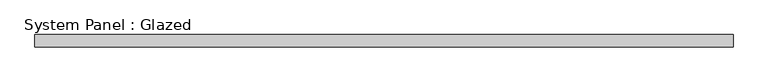
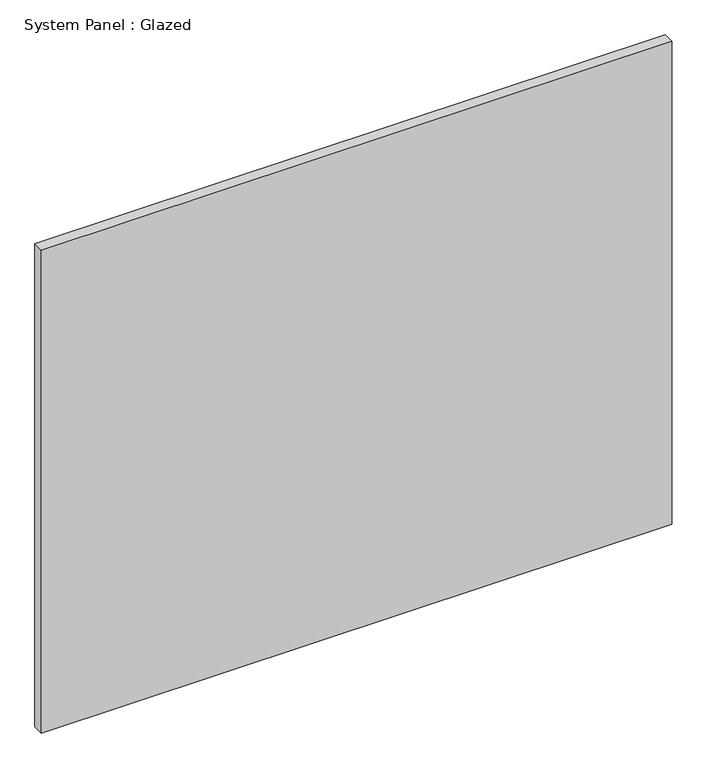
"""IFC4 building model written with IfcOpenShell, lengths in millimetres: plate geometry, System Panel : Glazed."""

import ifcopenshell
import ifcopenshell.guid

model = None  # the IFC model being written
_history = None  # IfcOwnerHistory: only IFC2X3 demands one
_inside = {}  # id of a spatial element -> (the spatial element, [elements in it])
_under = {}  # id of a project, library or spatial element -> (it, [spatial elements below it])
_declared = {}  # id of a project -> (the project, [libraries it declares])
_typed = {}  # id of a type object -> (the type object, [elements of that type])
_made_of = {}  # id of a material, layer set ... -> (it, [elements and type objects made of it])


def new_model(schema):
    """Start an empty IFC model of exactly this schema.

    Asked for "IFC4X3", IfcOpenShell would pick the latest addendum, in which some entities
    have other attributes; the version numbers below select the first issue.
    IFC2X3 requires an IfcOwnerHistory on every rooted entity: one is made here for all.
    """
    global model, _history
    if schema == "IFC4X3":
        model = ifcopenshell.file(schema_version=(4, 3, 0, 0))
    else:
        model = ifcopenshell.file(schema=schema)
    _inside.clear()
    _under.clear()
    _declared.clear()
    _typed.clear()
    _made_of.clear()
    _history = None
    if model.schema == "IFC2X3":
        org = make("IfcOrganization", Name="unknown")
        user = make(
            "IfcPersonAndOrganization",
            ThePerson=make("IfcPerson", FamilyName="unknown"),
            TheOrganization=org,
        )
        app = make(
            "IfcApplication",
            ApplicationDeveloper=org,
            Version="unknown",
            ApplicationFullName="unknown",
            ApplicationIdentifier="unknown",
        )
        _history = make(
            "IfcOwnerHistory",
            OwningUser=user,
            OwningApplication=app,
            ChangeAction="ADDED",
            CreationDate=0,
        )
    return model


def make(cls, **values):
    """One entity of the class cls with the attributes given. An attribute that is None is left unset."""
    return model.create_entity(
        cls, **{name: value for name, value in values.items() if value is not None}
    )


def rooted(cls, **values):
    """An entity with a GlobalId (a new one), such as an element, a storey or a relation."""
    return make(cls, GlobalId=ifcopenshell.guid.new(), OwnerHistory=_history, **values)


def si_unit(unit_type, name, prefix=None):
    """IfcSIUnit, for example si_unit("LENGTHUNIT", "METRE", prefix="MILLI")."""
    return make("IfcSIUnit", UnitType=unit_type, Prefix=prefix, Name=name)


def assignment(units):
    """IfcUnitAssignment: the units of a project."""
    return None if units is None else make("IfcUnitAssignment", Units=units)


def point(xyz):
    """IfcCartesianPoint."""
    return None if xyz is None else make("IfcCartesianPoint", Coordinates=xyz)


def direction(xyz):
    """IfcDirection."""
    return None if xyz is None else make("IfcDirection", DirectionRatios=xyz)


def frame(location, z_axis=None, x_axis=None):
    """IfcAxis2Placement3D, a coordinate frame: its origin and axes. An axis left out is left unset."""
    return make(
        "IfcAxis2Placement3D",
        Location=point(location),
        Axis=direction(z_axis),
        RefDirection=direction(x_axis),
    )


def origin():
    """The frame at (0, 0, 0) with its axes left unset."""
    return frame((0.0, 0.0, 0.0))


def origin_with_axes():
    """The frame at (0, 0, 0) with the z axis (0, 0, 1) and the x axis (1, 0, 0) written out."""
    return frame((0.0, 0.0, 0.0), z_axis=(0.0, 0.0, 1.0), x_axis=(1.0, 0.0, 0.0))


def place(relative_to, where):
    """IfcLocalPlacement: puts the frame where relative to a parent placement (None: the world)."""
    return make(
        "IfcLocalPlacement", PlacementRelTo=relative_to, RelativePlacement=where
    )


def context(
    kind, dimensions, precision=None, world=None, true_north=None, identifier=None
):
    """IfcGeometricRepresentationContext, for example the 3D "Model" context."""
    return make(
        "IfcGeometricRepresentationContext",
        ContextIdentifier=identifier,
        ContextType=kind,
        CoordinateSpaceDimension=dimensions,
        Precision=precision,
        WorldCoordinateSystem=world,
        TrueNorth=true_north,
    )


def project(units=None, contexts=None):
    """IfcProject with its units and contexts."""
    return rooted(
        "IfcProject",
        Name="project",
        RepresentationContexts=contexts,
        UnitsInContext=assignment(units),
    )


def spatial(cls, under=None, at=None, **own):
    """A site, building, storey or space (cls), placed at a placement, below another one or the project."""
    s = rooted(cls, ObjectPlacement=at, **own)
    if under is not None:
        _under.setdefault(under.id(), (under, []))[1].append(s)
    return s


def polyline(points):
    """IfcPolyline through the points."""
    return make("IfcPolyline", Points=[point(p) for p in points])


def outline(outer, holes=None, kind="AREA"):
    """IfcArbitraryClosedProfileDef: a profile drawn as a closed curve; with holes, ...WithVoids."""
    if holes is None:
        return make("IfcArbitraryClosedProfileDef", ProfileType=kind, OuterCurve=outer)
    return make(
        "IfcArbitraryProfileDefWithVoids",
        ProfileType=kind,
        OuterCurve=outer,
        InnerCurves=holes,
    )


def extrude(swept, where, along, depth):
    """IfcExtrudedAreaSolid: the profile swept, set in the frame where, extruded along a direction by depth."""
    return make(
        "IfcExtrudedAreaSolid",
        SweptArea=swept,
        Position=where,
        ExtrudedDirection=direction(along),
        Depth=depth,
    )


def shape(context_of_items, identifier, shape_type, items):
    """IfcShapeRepresentation: the items that make up one representation, for example the "Body"."""
    return make(
        "IfcShapeRepresentation",
        ContextOfItems=context_of_items,
        RepresentationIdentifier=identifier,
        RepresentationType=shape_type,
        Items=items,
    )


def source(mapping_origin, context_of_items, identifier, shape_type, items):
    """IfcRepresentationMap: a shape defined once, which mapped items show again and again."""
    return make(
        "IfcRepresentationMap",
        MappingOrigin=mapping_origin,
        MappedRepresentation=shape(context_of_items, identifier, shape_type, items),
    )


def transform(
    local_origin,
    x_axis=None,
    y_axis=None,
    z_axis=None,
    scale=None,
    scale2=None,
    scale3=None,
    uniform=True,
):
    """IfcCartesianTransformationOperator3D, or its non-uniform kind. x_axis, y_axis, z_axis: its Axis1, 2, 3."""
    if uniform:
        return make(
            "IfcCartesianTransformationOperator3D",
            Axis1=direction(x_axis),
            Axis2=direction(y_axis),
            LocalOrigin=point(local_origin),
            Scale=scale,
            Axis3=direction(z_axis),
        )
    return make(
        "IfcCartesianTransformationOperator3DnonUniform",
        Axis1=direction(x_axis),
        Axis2=direction(y_axis),
        LocalOrigin=point(local_origin),
        Scale=scale,
        Axis3=direction(z_axis),
        Scale2=scale2,
        Scale3=scale3,
    )


def mapped(mapping_source, mapping_target):
    """IfcMappedItem: shows the shape of a source again, moved by a transform."""
    return make(
        "IfcMappedItem", MappingSource=mapping_source, MappingTarget=mapping_target
    )


def made_of(thing, what):
    """Note that an element or type object is made of a material, layer set ...; save() writes the relation."""
    if what is not None:
        _made_of.setdefault(what.id(), (what, []))[1].append(thing)
    return thing


def element(
    cls,
    number,
    at=None,
    inside=None,
    cuts=None,
    type_object=None,
    material=None,
    context=None,
    identifier="Body",
    shape_type=None,
    held_by="IfcProductDefinitionShape",
    body=None,
    shapes=None,
    **own,
):
    """One element of the class cls, such as IfcWall. Its Tag is "e" and its number.

    at: its placement. inside: the storey or other place that contains it. cuts: it is an
    opening in that element (IfcRelVoidsElement). A single representation is given by context,
    identifier, shape_type and body (its items); several are given by shapes. held_by: the class
    of the entity that holds the representations. save() writes the other relations.
    """
    e = rooted(cls, Tag="e%d" % number, ObjectPlacement=at, **own)
    if body is not None:
        shapes = [shape(context, identifier, shape_type, body)]
    if shapes is not None:
        e.Representation = make(held_by, Representations=shapes)
    if inside is not None:
        _inside.setdefault(inside.id(), (inside, []))[1].append(e)
    if cuts is not None:
        rooted(
            "IfcRelVoidsElement", RelatingBuildingElement=cuts, RelatedOpeningElement=e
        )
    if type_object is not None:
        _typed.setdefault(type_object.id(), (type_object, []))[1].append(e)
    return made_of(e, material)


def aggregate(whole, parts):
    """IfcRelAggregates: a whole, such as a stair, and the parts it consists of."""
    return rooted("IfcRelAggregates", RelatingObject=whole, RelatedObjects=parts)


def save(model, path):
    """Write the relations noted so far, then the file.

    IfcRelAggregates (storeys below a building ...), IfcRelContainedInSpatialStructure (elements
    in a storey), IfcRelDefinesByType, IfcRelAssociatesMaterial and IfcRelDeclares: one each for
    every whole, place, type object, material and project.
    """
    for whole, parts in _under.values():
        aggregate(whole, parts)
    for where, things in _inside.values():
        rooted(
            "IfcRelContainedInSpatialStructure",
            RelatedElements=things,
            RelatingStructure=where,
        )
    for kind, things in _typed.values():
        rooted("IfcRelDefinesByType", RelatedObjects=things, RelatingType=kind)
    for what, things in _made_of.values():
        rooted("IfcRelAssociatesMaterial", RelatedObjects=things, RelatingMaterial=what)
    for by, libraries in _declared.values():
        rooted("IfcRelDeclares", RelatingContext=by, RelatedDefinitions=libraries)
    model.write(path)


def system_panel_glazed_8e8b8cb0(model_context):
    return source(origin(), model_context, "Body", "SweptSolid", [
        extrude(outline(polyline([(713.3166666, 19.05), (-713.3166666, 19.05), (-713.3166666, 44.45), (713.3166666, 44.45), (713.3166666, 19.05)])), origin_with_axes(), (0.0, 0.0, 1.0), 1155.7),
    ])


if __name__ == "__main__":
    model = new_model("IFC4")
    model_context = context("Model", 3, world=origin())
    ifc_project = project(units=[si_unit("LENGTHUNIT", "METRE", prefix="MILLI")], contexts=[model_context])
    site = spatial("IfcSite", under=ifc_project)
    building = spatial("IfcBuilding", under=site)
    placement = place(None, origin())
    system_panel_glazed_shape = system_panel_glazed_8e8b8cb0(model_context)
    element("IfcPlate", 1, ObjectType="System Panel : Glazed", at=placement, inside=building, context=model_context, shape_type="MappedRepresentation", body=[
        mapped(system_panel_glazed_shape, transform((0.0, 0.0, 0.0), x_axis=(1.0, 0.0, 0.0), y_axis=(0.0, 1.0, 0.0), z_axis=(0.0, 0.0, 1.0))),
    ])
    save(model, "model.ifc")

# Revit data of these elements
# Type "System Panel : Glazed"
#   Construction Type Id = "GSP4R"
#   Analytic Construction = "1/8 in Pilkington single glazing"
#   Visual Light Transmittance = 0.9
#   Solar Heat Gain Coefficient = 0.86
#   Heat Transfer Coefficient (U) = 1.18115 BTU/(h·ft²·°F)
#   Define Thermal Properties by = 1
# Element 1 (IfcPlate, "System Panel : Glazed")
#   Materials on its faces: "Glass"
# Materials
#   "Glass": class "Glass", colour RGB 0 128 192, transparency 0.75, Description = "Soda Lime Glass", Cost = 0
